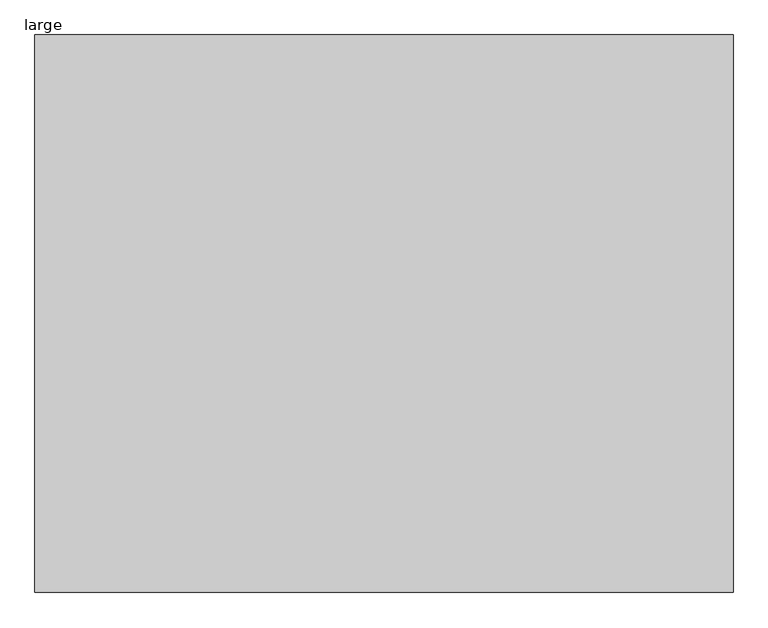
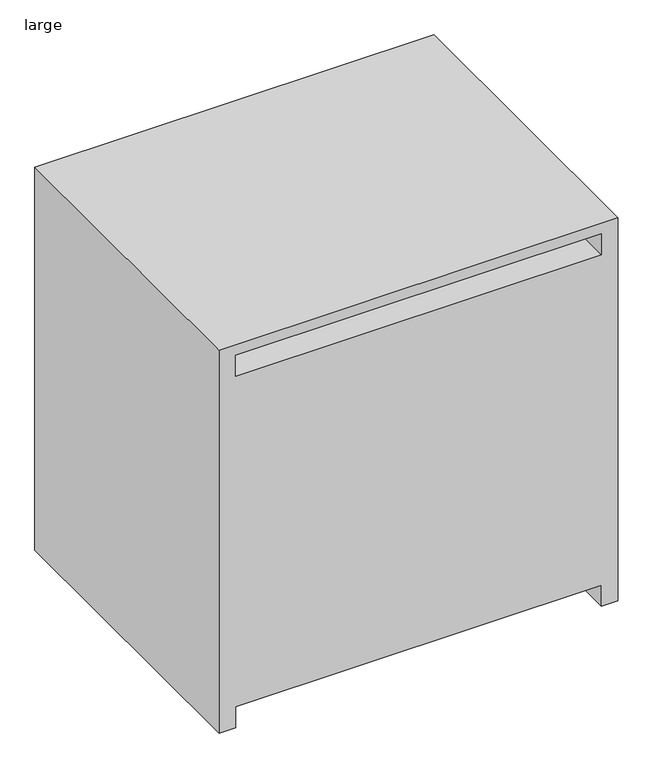
"""IFC4 building model written with IfcOpenShell, lengths in millimetres: proxy geometry, Transformer-Dry-Type-Siemens : large."""

import ifcopenshell
import ifcopenshell.guid

model = None  # the IFC model being written
_history = None  # IfcOwnerHistory: only IFC2X3 demands one
_inside = {}  # id of a spatial element -> (the spatial element, [elements in it])
_under = {}  # id of a project, library or spatial element -> (it, [spatial elements below it])
_declared = {}  # id of a project -> (the project, [libraries it declares])
_typed = {}  # id of a type object -> (the type object, [elements of that type])
_made_of = {}  # id of a material, layer set ... -> (it, [elements and type objects made of it])


def new_model(schema):
    """Start an empty IFC model of exactly this schema.

    Asked for "IFC4X3", IfcOpenShell would pick the latest addendum, in which some entities
    have other attributes; the version numbers below select the first issue.
    IFC2X3 requires an IfcOwnerHistory on every rooted entity: one is made here for all.
    """
    global model, _history
    if schema == "IFC4X3":
        model = ifcopenshell.file(schema_version=(4, 3, 0, 0))
    else:
        model = ifcopenshell.file(schema=schema)
    _inside.clear()
    _under.clear()
    _declared.clear()
    _typed.clear()
    _made_of.clear()
    _history = None
    if model.schema == "IFC2X3":
        org = make("IfcOrganization", Name="unknown")
        user = make(
            "IfcPersonAndOrganization",
            ThePerson=make("IfcPerson", FamilyName="unknown"),
            TheOrganization=org,
        )
        app = make(
            "IfcApplication",
            ApplicationDeveloper=org,
            Version="unknown",
            ApplicationFullName="unknown",
            ApplicationIdentifier="unknown",
        )
        _history = make(
            "IfcOwnerHistory",
            OwningUser=user,
            OwningApplication=app,
            ChangeAction="ADDED",
            CreationDate=0,
        )
    return model


def make(cls, **values):
    """One entity of the class cls with the attributes given. An attribute that is None is left unset."""
    return model.create_entity(
        cls, **{name: value for name, value in values.items() if value is not None}
    )


def rooted(cls, **values):
    """An entity with a GlobalId (a new one), such as an element, a storey or a relation."""
    return make(cls, GlobalId=ifcopenshell.guid.new(), OwnerHistory=_history, **values)


def si_unit(unit_type, name, prefix=None):
    """IfcSIUnit, for example si_unit("LENGTHUNIT", "METRE", prefix="MILLI")."""
    return make("IfcSIUnit", UnitType=unit_type, Prefix=prefix, Name=name)


def assignment(units):
    """IfcUnitAssignment: the units of a project."""
    return None if units is None else make("IfcUnitAssignment", Units=units)


def point(xyz):
    """IfcCartesianPoint."""
    return None if xyz is None else make("IfcCartesianPoint", Coordinates=xyz)


def direction(xyz):
    """IfcDirection."""
    return None if xyz is None else make("IfcDirection", DirectionRatios=xyz)


def frame(location, z_axis=None, x_axis=None):
    """IfcAxis2Placement3D, a coordinate frame: its origin and axes. An axis left out is left unset."""
    return make(
        "IfcAxis2Placement3D",
        Location=point(location),
        Axis=direction(z_axis),
        RefDirection=direction(x_axis),
    )


def origin():
    """The frame at (0, 0, 0) with its axes left unset."""
    return frame((0.0, 0.0, 0.0))


def place(relative_to, where):
    """IfcLocalPlacement: puts the frame where relative to a parent placement (None: the world)."""
    return make(
        "IfcLocalPlacement", PlacementRelTo=relative_to, RelativePlacement=where
    )


def context(
    kind, dimensions, precision=None, world=None, true_north=None, identifier=None
):
    """IfcGeometricRepresentationContext, for example the 3D "Model" context."""
    return make(
        "IfcGeometricRepresentationContext",
        ContextIdentifier=identifier,
        ContextType=kind,
        CoordinateSpaceDimension=dimensions,
        Precision=precision,
        WorldCoordinateSystem=world,
        TrueNorth=true_north,
    )


def project(units=None, contexts=None):
    """IfcProject with its units and contexts."""
    return rooted(
        "IfcProject",
        Name="project",
        RepresentationContexts=contexts,
        UnitsInContext=assignment(units),
    )


def spatial(cls, under=None, at=None, **own):
    """A site, building, storey or space (cls), placed at a placement, below another one or the project."""
    s = rooted(cls, ObjectPlacement=at, **own)
    if under is not None:
        _under.setdefault(under.id(), (under, []))[1].append(s)
    return s


def polyline(points):
    """IfcPolyline through the points."""
    return make("IfcPolyline", Points=[point(p) for p in points])


def outline(outer, holes=None, kind="AREA"):
    """IfcArbitraryClosedProfileDef: a profile drawn as a closed curve; with holes, ...WithVoids."""
    if holes is None:
        return make("IfcArbitraryClosedProfileDef", ProfileType=kind, OuterCurve=outer)
    return make(
        "IfcArbitraryProfileDefWithVoids",
        ProfileType=kind,
        OuterCurve=outer,
        InnerCurves=holes,
    )


def extrude(swept, where, along, depth):
    """IfcExtrudedAreaSolid: the profile swept, set in the frame where, extruded along a direction by depth."""
    return make(
        "IfcExtrudedAreaSolid",
        SweptArea=swept,
        Position=where,
        ExtrudedDirection=direction(along),
        Depth=depth,
    )


def shape(context_of_items, identifier, shape_type, items):
    """IfcShapeRepresentation: the items that make up one representation, for example the "Body"."""
    return make(
        "IfcShapeRepresentation",
        ContextOfItems=context_of_items,
        RepresentationIdentifier=identifier,
        RepresentationType=shape_type,
        Items=items,
    )


def source(mapping_origin, context_of_items, identifier, shape_type, items):
    """IfcRepresentationMap: a shape defined once, which mapped items show again and again."""
    return make(
        "IfcRepresentationMap",
        MappingOrigin=mapping_origin,
        MappedRepresentation=shape(context_of_items, identifier, shape_type, items),
    )


def transform(
    local_origin,
    x_axis=None,
    y_axis=None,
    z_axis=None,
    scale=None,
    scale2=None,
    scale3=None,
    uniform=True,
):
    """IfcCartesianTransformationOperator3D, or its non-uniform kind. x_axis, y_axis, z_axis: its Axis1, 2, 3."""
    if uniform:
        return make(
            "IfcCartesianTransformationOperator3D",
            Axis1=direction(x_axis),
            Axis2=direction(y_axis),
            LocalOrigin=point(local_origin),
            Scale=scale,
            Axis3=direction(z_axis),
        )
    return make(
        "IfcCartesianTransformationOperator3DnonUniform",
        Axis1=direction(x_axis),
        Axis2=direction(y_axis),
        LocalOrigin=point(local_origin),
        Scale=scale,
        Axis3=direction(z_axis),
        Scale2=scale2,
        Scale3=scale3,
    )


def mapped(mapping_source, mapping_target):
    """IfcMappedItem: shows the shape of a source again, moved by a transform."""
    return make(
        "IfcMappedItem", MappingSource=mapping_source, MappingTarget=mapping_target
    )


def made_of(thing, what):
    """Note that an element or type object is made of a material, layer set ...; save() writes the relation."""
    if what is not None:
        _made_of.setdefault(what.id(), (what, []))[1].append(thing)
    return thing


def element(
    cls,
    number,
    at=None,
    inside=None,
    cuts=None,
    type_object=None,
    material=None,
    context=None,
    identifier="Body",
    shape_type=None,
    held_by="IfcProductDefinitionShape",
    body=None,
    shapes=None,
    **own,
):
    """One element of the class cls, such as IfcWall. Its Tag is "e" and its number.

    at: its placement. inside: the storey or other place that contains it. cuts: it is an
    opening in that element (IfcRelVoidsElement). A single representation is given by context,
    identifier, shape_type and body (its items); several are given by shapes. held_by: the class
    of the entity that holds the representations. save() writes the other relations.
    """
    e = rooted(cls, Tag="e%d" % number, ObjectPlacement=at, **own)
    if body is not None:
        shapes = [shape(context, identifier, shape_type, body)]
    if shapes is not None:
        e.Representation = make(held_by, Representations=shapes)
    if inside is not None:
        _inside.setdefault(inside.id(), (inside, []))[1].append(e)
    if cuts is not None:
        rooted(
            "IfcRelVoidsElement", RelatingBuildingElement=cuts, RelatedOpeningElement=e
        )
    if type_object is not None:
        _typed.setdefault(type_object.id(), (type_object, []))[1].append(e)
    return made_of(e, material)


def aggregate(whole, parts):
    """IfcRelAggregates: a whole, such as a stair, and the parts it consists of."""
    return rooted("IfcRelAggregates", RelatingObject=whole, RelatedObjects=parts)


def save(model, path):
    """Write the relations noted so far, then the file.

    IfcRelAggregates (storeys below a building ...), IfcRelContainedInSpatialStructure (elements
    in a storey), IfcRelDefinesByType, IfcRelAssociatesMaterial and IfcRelDeclares: one each for
    every whole, place, type object, material and project.
    """
    for whole, parts in _under.values():
        aggregate(whole, parts)
    for where, things in _inside.values():
        rooted(
            "IfcRelContainedInSpatialStructure",
            RelatedElements=things,
            RelatingStructure=where,
        )
    for kind, things in _typed.values():
        rooted("IfcRelDefinesByType", RelatedObjects=things, RelatingType=kind)
    for what, things in _made_of.values():
        rooted("IfcRelAssociatesMaterial", RelatedObjects=things, RelatingMaterial=what)
    for by, libraries in _declared.values():
        rooted("IfcRelDeclares", RelatingContext=by, RelatedDefinitions=libraries)
    model.write(path)


def large_8446dd82(model_context):
    return source(origin(), model_context, "Body", "SweptSolid", [
        extrude(outline(polyline([(1854.2, 914.4), (1854.2, -914.4), (0.0, -914.4), (0.0, -838.2), (101.6, -838.2), (101.6, 838.2), (0.0, 838.2), (0.0, 914.4), (1854.2, 914.4)]), holes=[polyline([(1803.4, 838.2), (1701.8, 838.2), (1701.8, -838.2), (1803.4, -838.2), (1803.4, 838.2)])]), frame((0.0, -730.25, 0.0), z_axis=(0.0, 1.0, 0.0), x_axis=(0.0, 0.0, 1.0)), (0.0, 0.0, 1.0), 1460.5),
    ])


if __name__ == "__main__":
    model = new_model("IFC4")
    model_context = context("Model", 3, world=origin())
    ifc_project = project(units=[si_unit("LENGTHUNIT", "METRE", prefix="MILLI")], contexts=[model_context])
    site = spatial("IfcSite", under=ifc_project)
    building = spatial("IfcBuilding", under=site)
    placement = place(None, origin())
    large_shape = large_8446dd82(model_context)
    element("IfcBuildingElementProxy", 1, Name="Transformer-Dry-Type-Siemens : large", ObjectType="Transformer-Dry-Type-Siemens : large", at=placement, inside=building, context=model_context, shape_type="MappedRepresentation", body=[
        mapped(large_shape, transform((0.0, 0.0, 0.0), x_axis=(1.0, 0.0, 0.0), y_axis=(0.0, 1.0, 0.0), z_axis=(0.0, 0.0, 1.0))),
    ])
    save(model, "model.ifc")

# Revit data of these elements
# Type "Transformer-Dry-Type-Siemens : large"
#   Weight = "5500"
#   Wattage = "DO NOT USE"
#   Voltage = "DO NOT USE"
#   URL = "http://www.usa.siemens.com/ce"
#   Transformer Material = "Aluminum"
#   Product Page URL = "http://www.sea.siemens.com/us/Products/PowerDistribution/Product/Transformers/Pages/Transformers.aspx"
#   Product Documentation Link = "http://www.sea.siemens.com/us/internet-dms/Internet/ConsultingEngineersComm/General/Docs/drytrans.pdf"
#   Model = "3F3Y015K13TP1"
#   Manufacturer = "Siemens Industry"
#   KVA = "750"
#   K Factor = "13"
#   Description = "Transformer"
#   Deg Rise = "150"
#   Copyright © = "© Siemens Industry, Inc. 2011"
#   CTRL Connector Description = "Equipment Power"
#   BOM URL [instance default] = ""
#   Assembly Code = "D5090900"
#   clearance = 3' - 0"
#   Width = 6' - 0"
#   Primary Voltage = 480 V
#   Power Factor = 1
#   Height = 6' - 1"
#   Depth = 4' - 9 1/2"
#   Apparent Load [instance default] = 0 VA
#   Has Not Contacted Siemens For Configuration [instance default] = no
#   Contacted Siemens For Configuration [instance default] = yes
#   Text Material = Paint- Siemens - Dark
#   Frame Material = ELECTRICAL TRANSFORMERS
# Element 1 (IfcBuildingElementProxy, "Transformer-Dry-Type-Siemens : large")
#   Materials on its faces: "ELECTRICAL TRANSFORMERS"
# Materials
#   "Paint- Siemens - Dark": class "Metal", colour RGB 175 38 68, transparency 0
#   "ELECTRICAL TRANSFORMERS": class "Metal", colour RGB 63 114 97, transparency 0, Cost = 0
